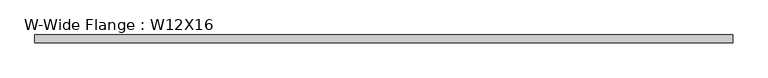
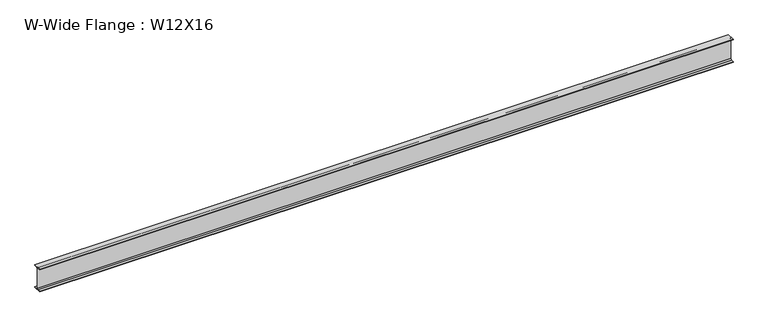
"""IFC4 building model written with IfcOpenShell, lengths in millimetres: beam geometry, W-Wide Flange : W12X16."""

from ifc_helpers import new_model, si_unit, point, frame, frame_2d, origin, place, context, project, spatial, polyline, circle_curve, trimmed, segment, composite_curve, outline, extrude, source, transform, mapped, element, save


def w_wide_flange_w12x16_ddd03c39(model_context):
    return source(origin(), model_context, "Body", "SweptSolid", [
        extrude(outline(composite_curve([segment(polyline([(50.673, -145.669), (50.673, -152.4), (-50.673, -152.4), (-50.673, -145.669), (-16.7005, -145.669)]), True, "CONTINUOUS"), segment(trimmed(circle_curve(frame_2d((-16.7005, -131.7625)), 13.9065), [point((-16.7005, -145.669))], [point((-2.794, -131.7625))], True, "CARTESIAN"), True, "CONTINUOUS"), segment(polyline([(-2.794, -131.7625), (-2.794, 131.7625)]), True, "CONTINUOUS"), segment(trimmed(circle_curve(frame_2d((-16.7005, 131.7625)), 13.9065), [point((-2.794, 131.7625))], [point((-16.7005, 145.669))], True, "CARTESIAN"), True, "CONTINUOUS"), segment(polyline([(-16.7005, 145.669), (-50.673, 145.669), (-50.673, 152.4), (50.673, 152.4), (50.673, 145.669), (16.7005, 145.669)]), True, "CONTINUOUS"), segment(trimmed(circle_curve(frame_2d((16.7005, 131.7625)), 13.9065), [point((16.7005, 145.669))], [point((2.794, 131.7625))], True, "CARTESIAN"), True, "CONTINUOUS"), segment(polyline([(2.794, 131.7625), (2.794, -131.7625)]), True, "CONTINUOUS"), segment(trimmed(circle_curve(frame_2d((16.7005, -131.7625)), 13.9065), [point((2.794, -131.7625))], [point((16.7005, -145.669))], True, "CARTESIAN"), True, "CONTINUOUS"), segment(polyline([(16.7005, -145.669), (50.673, -145.669)]), True, "CONTINUOUS")], self_intersect=False)), frame((-4381.4503906, 0.0, 0.0), z_axis=(1.0, 0.0, 0.0), x_axis=(0.0, 1.0, 0.0)), (0.0, 0.0, 1.0), 8839.1007812),
    ])


if __name__ == "__main__":
    model = new_model("IFC4")
    model_context = context("Model", 3, world=origin())
    ifc_project = project(units=[si_unit("LENGTHUNIT", "METRE", prefix="MILLI")], contexts=[model_context])
    site = spatial("IfcSite", under=ifc_project)
    building = spatial("IfcBuilding", under=site)
    placement = place(None, origin())
    w_wide_flange_w12x16_shape = w_wide_flange_w12x16_ddd03c39(model_context)
    element("IfcBeam", 1, ObjectType="W-Wide Flange : W12X16", at=placement, inside=building, context=model_context, shape_type="MappedRepresentation", body=[
        mapped(w_wide_flange_w12x16_shape, transform((0.0, 0.0, 0.0), x_axis=(1.0, 0.0, 0.0), y_axis=(0.0, 1.0, 0.0), z_axis=(0.0, 0.0, 1.0))),
    ])
    save(model, "model.ifc")

# Revit data of these elements
# Type "W-Wide Flange : W12X16"
#   Assembly Code = "B10"
#   W = 16
#   Length [instance default] = 1524 mm
#   bf = 101.346 mm
#   d = 304.8 mm
#   k = 20.638 mm
#   k2 = 13.907 mm
#   tf = 6.731 mm
#   tw = 5.588 mm
#   A = 0.0030387 m²
#   Structural Material [instance default] = Steel ASTM A992
# Element 1 (IfcBeam, "W-Wide Flange : W12X16")
#   Structural Material = Aluminum, Anodized Red
#   Materials on its faces: "Aluminum, Anodized Red"
# Materials
#   "Steel ASTM A992": class "Metal", colour RGB 128 0 0, transparency 0, Description = "Structural steel 50ksi", Cost = 0
#   "Aluminum, Anodized Red": class "Metal", colour RGB 120 120 120, transparency 0, Description = "Anodized aluminum, red", Cost = 0
